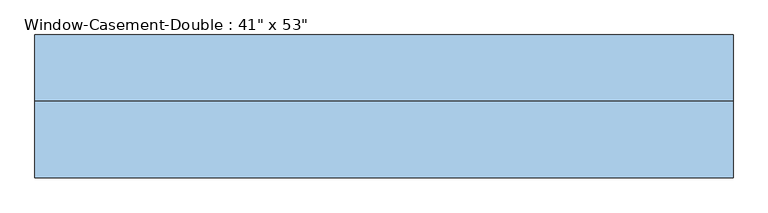
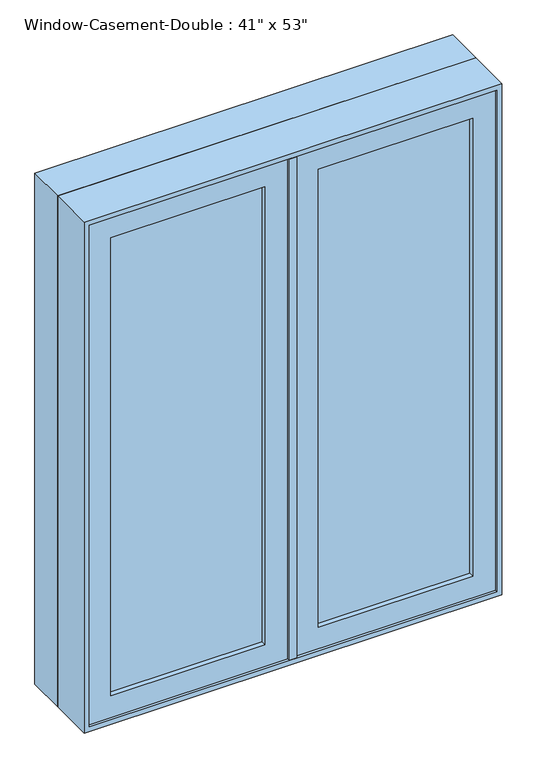
"""IFC4 building model written with IfcOpenShell, lengths in millimetres: window geometry."""

from ifc_helpers import new_model, si_unit, frame, origin, place, context, project, spatial, polyline, outline, extrude, faceted_brep, source, transform, mapped, element, save


def window_54fa335d(model_context):
    return source(origin(), model_context, "Body", "SolidModel", [
        faceted_brep([(9.525, -115.8875, 2247.9), (9.525, -65.0875, 2247.9), (-9.525, -65.0875, 2247.9), (-9.525, -115.8875, 2247.9), (9.525, -115.8875, 927.1), (-9.525, -115.8875, 927.1), (-9.525, -65.0875, 927.1), (9.525, -65.0875, 927.1), (-9.525, -65.0875, 2228.85), (-9.525, -65.0875, 946.15), (-30.1625, -65.0875, 2228.85), (-30.1625, -65.0875, 946.15), (-30.1625, -1.5875, 2228.85), (-30.1625, -1.5875, 946.15), (30.1625, -1.5875, 2228.85), (30.1625, -1.5875, 946.15), (30.1625, -65.0875, 2228.85), (30.1625, -65.0875, 946.15), (9.525, -65.0875, 2228.85), (9.525, -65.0875, 946.15)], [[[0, 1, 2, 3]], [[4, 5, 6, 7]], [[3, 5, 4, 0]], [[2, 8, 9, 6, 5, 3]], [[8, 10, 11, 9]], [[10, 12, 13, 11]], [[12, 14, 15, 13]], [[14, 16, 17, 15]], [[16, 18, 19, 17]], [[0, 4, 7, 19, 18, 1]], [[8, 2, 1, 18]], [[19, 7, 6, 9]], [[9, 11, 13, 15, 17, 19]], [[18, 16, 14, 12, 10, 8]]]),
        extrude(outline(polyline([(-66.675, -96.8375), (-450.85, -96.8375), (-450.85, -90.4875), (-66.675, -90.4875), (-66.675, -96.8375)])), frame((0.0, 0.0, 984.25), z_axis=(0.0, 0.0, 1.0), x_axis=(1.0, 0.0, 0.0)), (0.0, 0.0, 1.0), 1206.5),
        extrude(outline(polyline([(-450.85, -77.7875), (-66.675, -77.7875), (-66.675, -84.1375), (-450.85, -84.1375), (-450.85, -77.7875)])), frame((0.0, 0.0, 984.25), z_axis=(0.0, 0.0, 1.0), x_axis=(1.0, 0.0, 0.0)), (0.0, 0.0, 1.0), 1206.5),
        extrude(outline(polyline([(450.85, -96.8375), (66.675, -96.8375), (66.675, -90.4875), (450.85, -90.4875), (450.85, -96.8375)])), frame((0.0, 0.0, 984.25), z_axis=(0.0, 0.0, 1.0), x_axis=(1.0, 0.0, 0.0)), (0.0, 0.0, 1.0), 1206.5),
        extrude(outline(polyline([(66.675, -77.7875), (450.85, -77.7875), (450.85, -84.1375), (66.675, -84.1375), (66.675, -77.7875)])), frame((0.0, 0.0, 984.25), z_axis=(0.0, 0.0, 1.0), x_axis=(1.0, 0.0, 0.0)), (0.0, 0.0, 1.0), 1206.5),
        extrude(outline(polyline([(2247.9, -9.525), (2247.9, -508.0), (927.1, -508.0), (927.1, -9.525), (2247.9, -9.525)]), holes=[polyline([(2190.75, -450.85), (2190.75, -66.675), (984.25, -66.675), (984.25, -450.85), (2190.75, -450.85)])]), frame((0.0, -109.5375, 0.0), z_axis=(0.0, 1.0, 0.0), x_axis=(0.0, 0.0, 1.0)), (0.0, 0.0, 1.0), 44.45),
        extrude(outline(polyline([(927.1, 9.525), (927.1, 508.0), (2247.9, 508.0), (2247.9, 9.525), (927.1, 9.525)]), holes=[polyline([(984.25, 450.85), (984.25, 66.675), (2190.75, 66.675), (2190.75, 450.85), (984.25, 450.85)])]), frame((0.0, -109.5375, 0.0), z_axis=(0.0, 1.0, 0.0), x_axis=(0.0, 0.0, 1.0)), (0.0, 0.0, 1.0), 44.45),
        extrude(outline(polyline([(2260.6, -520.7), (914.4, -520.7), (914.4, 520.7), (2260.6, 520.7), (2260.6, -520.7)]), holes=[polyline([(2241.55, 501.65), (933.45, 501.65), (933.45, -501.65), (2241.55, -501.65), (2241.55, 501.65)])]), frame((0.0, -1.5875, 0.0), z_axis=(0.0, 1.0, 0.0), x_axis=(0.0, 0.0, 1.0)), (0.0, 0.0, 1.0), 98.425),
        faceted_brep([(488.95, -65.0875, 2228.85), (-488.95, -65.0875, 2228.85), (-488.95, -1.5875, 2228.85), (488.95, -1.5875, 2228.85), (508.0, -115.8875, 2247.9), (-508.0, -115.8875, 2247.9), (-508.0, -65.0875, 2247.9), (508.0, -65.0875, 2247.9), (520.7, -1.5875, 2260.6), (-520.7, -1.5875, 2260.6), (-520.7, -115.8875, 2260.6), (520.7, -115.8875, 2260.6), (-488.95, -65.0875, 946.15), (-488.95, -1.5875, 946.15), (-508.0, -115.8875, 927.1), (-508.0, -65.0875, 927.1), (-520.7, -1.5875, 914.4), (-520.7, -115.8875, 914.4), (488.95, -65.0875, 946.15), (488.95, -1.5875, 946.15), (508.0, -115.8875, 927.1), (508.0, -65.0875, 927.1), (520.7, -1.5875, 914.4), (520.7, -115.8875, 914.4)], [[[0, 1, 2, 3]], [[4, 5, 6, 7]], [[8, 9, 10, 11]], [[1, 12, 13, 2]], [[5, 14, 15, 6]], [[9, 16, 17, 10]], [[12, 18, 19, 13]], [[14, 20, 21, 15]], [[16, 22, 23, 17]], [[9, 8, 22, 16], [3, 2, 13, 19]], [[18, 0, 3, 19]], [[7, 6, 15, 21], [1, 0, 18, 12]], [[20, 4, 7, 21]], [[22, 8, 11, 23]], [[11, 10, 17, 23], [5, 4, 20, 14]]]),
    ])


if __name__ == "__main__":
    model = new_model("IFC4")
    model_context = context("Model", 3, world=origin())
    ifc_project = project(units=[si_unit("LENGTHUNIT", "METRE", prefix="MILLI")], contexts=[model_context])
    site = spatial("IfcSite", under=ifc_project)
    building = spatial("IfcBuilding", under=site)
    placement = place(None, origin())
    window_shape = window_54fa335d(model_context)
    element("IfcWindow", 1, ObjectType="Window-Casement-Double : 41\" x 53\"", at=placement, inside=building, context=model_context, shape_type="MappedRepresentation", body=[
        mapped(window_shape, transform((0.0, 0.0, 0.0), x_axis=(1.0, 0.0, 0.0), y_axis=(0.0, 1.0, 0.0), z_axis=(0.0, 0.0, 1.0))),
    ])
    save(model, "model.ifc")

# Revit data of these elements
# Type "Window-Casement-Double : 41\" x 53\""
#   Type Mark = "60"
#   Fire Rating = "0.5h"
#   Assembly Code = "B2020100"
#   Analytic Construction = "Double glazing - domestic"
#   Frame Extension [instance default] = 0' - 0 1/4"
#   Window Inset [instance default] = 0' - 0"
#   Wall Thickness [instance default] = 0' - 6"
#   Interior Wall Closure [instance default] = 0' - 2 1/4"
#   Half Width = 1' - 8 1/2"
#   Visual Light Transmittance = 0.81
#   Thermal Resistance (R) = 1.8146 (h·ft²·°F)/BTU
#   Solar Heat Gain Coefficient = 0.76
#   Rough Width = 3' - 5 1/2"
#   Rough Height = 4' - 5 1/2"
#   Height = 4' - 5"
#   Heat Transfer Coefficient (U) = 0.5511 BTU/(h·ft²·°F)
#   Exterior Wall Closure [instance default] = 0' - 1 1/4"
#   Extension Jamb [instance default] = 0' - 2 1/4"
#   Default Sill Height = 3' - 0"
#   Width = 3' - 5"
#   Define Thermal Properties by = 0
#   Muntin Visibility = yes
#   Interior Trim Visibility [instance default] = yes
#   Exterior Trim Visibility [instance default] = yes
#   Extension Jamb Visibility [instance default] = yes
#   Interior Trim Material = Wood - Stained
#   Muntin Pattern = Muntin Pattern_2x2 : Muntin Pattern_2x2
#   Interior Trim = Trim-Window-Interior-Flat : Picture Frame
#   Interior Frame Material = Wood - Stained
#   Glass Panel Material = Glass
#   Exterior Trim Material = Clad - White
#   Exterior Trim = Trim-Window-Exterior-Flat : with Sill
#   Exterior Frame Material = Clad - White
#   Wall Closure = (empty or 0)
# Element 1 (IfcWindow, "Window-Casement-Double : 41\" x 53\"")
#   Wall Thickness = 0' - 7 5/8"
#   Extension Jamb = 0' - 3 7/8"
#   Materials on its faces: "Wood - Stained", "Glass", "Clad - White"
# Materials
#   "Wood - Stained": class "Wood", colour RGB 224 178 126, transparency 0, Cost = 0
#   "Glass": class "Glass", colour RGB 236 240 239, transparency 0.5, Description = "Soda Lime Glass", Cost = 0
#   "Clad - White": class "Wood", colour RGB 216 216 204, transparency 0, Cost = 0
